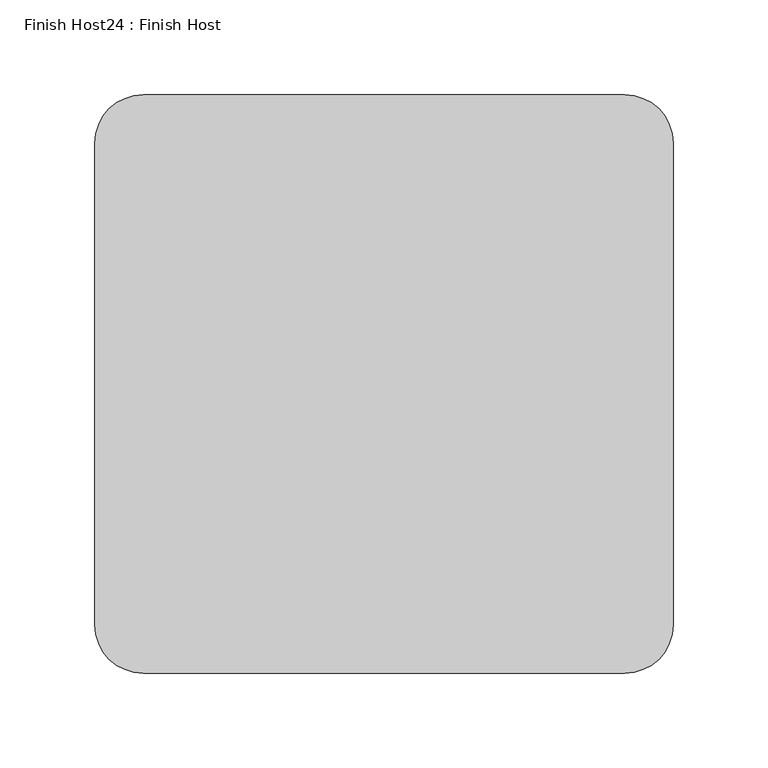
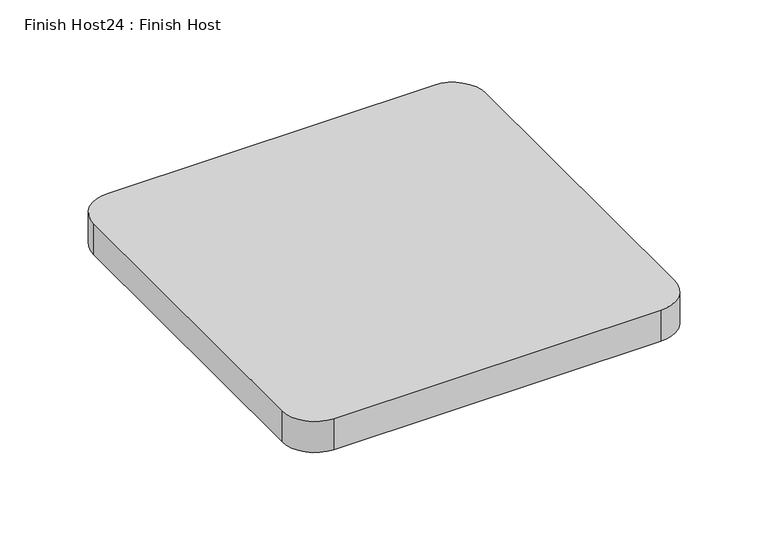
"""IFC4 building model written with IfcOpenShell, lengths in millimetres: proxy geometry, Finish Host24 : Finish Host."""

from ifc_helpers import new_model, si_unit, point, frame_2d, origin, origin_with_axes, place, context, project, spatial, polyline, circle_curve, trimmed, segment, composite_curve, outline, extrude, source, transform, mapped, element, save


def finish_host24_finish_host_ebc1b303(model_context):
    return source(origin(), model_context, "Body", "SweptSolid", [
        extrude(outline(composite_curve([segment(polyline([(-10878.637433, 8625.0675603), (-10878.637433, 8879.0675603)]), True, "CONTINUOUS"), segment(trimmed(circle_curve(frame_2d((-10853.237433, 8879.0675603)), 25.4), [point((-10878.637433, 8879.0675603))], [point((-10853.237433, 8904.4675603))], False, "CARTESIAN"), True, "CONTINUOUS"), segment(polyline([(-10853.237433, 8904.4675603), (-10599.237433, 8904.4675603)]), True, "CONTINUOUS"), segment(trimmed(circle_curve(frame_2d((-10599.237433, 8879.0675603)), 25.4), [point((-10599.237433, 8904.4675603))], [point((-10573.837433, 8879.0675603))], False, "CARTESIAN"), True, "CONTINUOUS"), segment(polyline([(-10573.837433, 8879.0675603), (-10573.837433, 8625.0675603)]), True, "CONTINUOUS"), segment(trimmed(circle_curve(frame_2d((-10599.237433, 8625.0675603)), 25.4), [point((-10573.837433, 8625.0675603))], [point((-10599.237433, 8599.6675603))], False, "CARTESIAN"), True, "CONTINUOUS"), segment(polyline([(-10599.237433, 8599.6675603), (-10853.237433, 8599.6675603)]), True, "CONTINUOUS"), segment(trimmed(circle_curve(frame_2d((-10853.237433, 8625.0675603)), 25.4), [point((-10853.237433, 8599.6675603))], [point((-10878.637433, 8625.0675603))], False, "CARTESIAN"), True, "CONTINUOUS")], self_intersect=False)), origin_with_axes(), (0.0, 0.0, 1.0), 25.4),
    ])


if __name__ == "__main__":
    model = new_model("IFC4")
    model_context = context("Model", 3, world=origin())
    ifc_project = project(units=[si_unit("LENGTHUNIT", "METRE", prefix="MILLI")], contexts=[model_context])
    site = spatial("IfcSite", under=ifc_project)
    building = spatial("IfcBuilding", under=site)
    placement = place(None, origin())
    finish_host24_finish_host_shape = finish_host24_finish_host_ebc1b303(model_context)
    element("IfcBuildingElementProxy", 1, Name="Finish Host24 : Finish Host", ObjectType="Finish Host24 : Finish Host", at=placement, inside=building, context=model_context, shape_type="MappedRepresentation", body=[
        mapped(finish_host24_finish_host_shape, transform((0.0, 0.0, 0.0), x_axis=(1.0, 0.0, 0.0), y_axis=(0.0, 1.0, 0.0), z_axis=(0.0, 0.0, 1.0))),
    ])
    save(model, "model.ifc")

# Revit data of these elements
# Type "Finish Host24 : Finish Host"
#   Panel Material = Fabric - Teknion - S610 - Saturate - Quarry
# Element 1 (IfcBuildingElementProxy, "Finish Host24 : Finish Host")
#   Materials on its faces: "Fabric - Teknion - S610 - Saturate - Quarry"
# Materials
#   "Fabric - Teknion - S610 - Saturate - Quarry": class "Fabric", colour RGB 43 43 44, transparency 0, Model = "S610", Manufacturer = "Teknion Studio", URL = "http://www.teknion.com/", Description = "Quarry Saturate", Cost = 0
